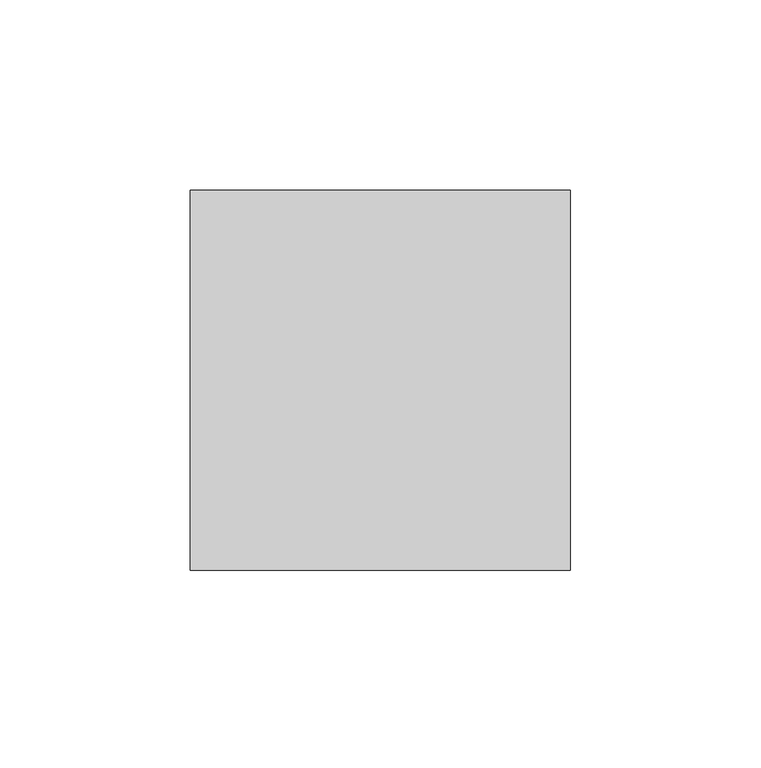
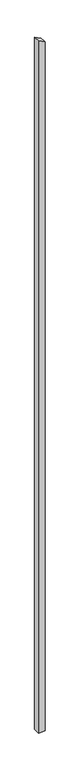
"""IFC4 building model written with IfcOpenShell, lengths in millimetres: column geometry, Holzstütze 158706 : Holzstütze 158706."""

from ifc_helpers import new_model, si_unit, frame, origin, place, context, project, spatial, polyline, outline, extrude, source, transform, mapped, element, save


def column_2f8b9505(model_context):
    return source(origin(), model_context, "Body", "SweptSolid", [
        extrude(outline(polyline([(-500.0, 165867.7593015), (-500.0, 165967.7593015), (10590.0588201, 165967.7593015), (10641.011365, 165867.7593015), (-500.0, 165867.7593015)])), frame((0.0, 47884.7962965, 0.0), z_axis=(0.0, 1.0, 0.0), x_axis=(0.0, 0.0, 1.0)), (0.0, 0.0, 1.0), 100.0),
    ])


if __name__ == "__main__":
    model = new_model("IFC4")
    model_context = context("Model", 3, world=origin())
    ifc_project = project(units=[si_unit("LENGTHUNIT", "METRE", prefix="MILLI")], contexts=[model_context])
    site = spatial("IfcSite", under=ifc_project)
    building = spatial("IfcBuilding", under=site)
    placement = place(None, origin())
    column_shape = column_2f8b9505(model_context)
    element("IfcColumn", 1, ObjectType="Holzstütze 158706 : Holzstütze 158706", at=placement, inside=building, context=model_context, shape_type="MappedRepresentation", body=[
        mapped(column_shape, transform((0.0, 0.0, 0.0), x_axis=(1.0, 0.0, 0.0), y_axis=(0.0, 1.0, 0.0), z_axis=(0.0, 0.0, 1.0))),
    ])
    save(model, "model.ifc")

# Revit data of these elements
# Type "Holzstütze 158706 : Holzstütze 158706"
#   Abrechnungsart = "m"
#   Allright_Bauteil_ID = "0152St 0000143525"
#   Bezeichnung = "Holzstütze"
#   Codetext = "ST-HOLZ\\"
#   Gewerk = "Zimmer- und Holzbauarbeiten"
#   Material = "Holz"
#   Objektname = "Stütze"
#   NameOverride = "Holzstütze"
#   Reference = "Holzstütze"
#   Status = "NEW"
#   ThermalTransmittance = 0.0000 BTU/(h·ft²·°F)
#   Roll = 0.00°
#   Slope = 0.00°
#   2D Interaktion = yes
#   IsExternal = yes
#   LoadBearing = yes
# Element 1 (IfcColumn, "Holzstütze 158706 : Holzstütze 158706")
#   Materials on its faces: "holzschalung"
# Materials
#   "holzschalung": class "Unassigned", colour RGB 128 128 128, transparency 0
